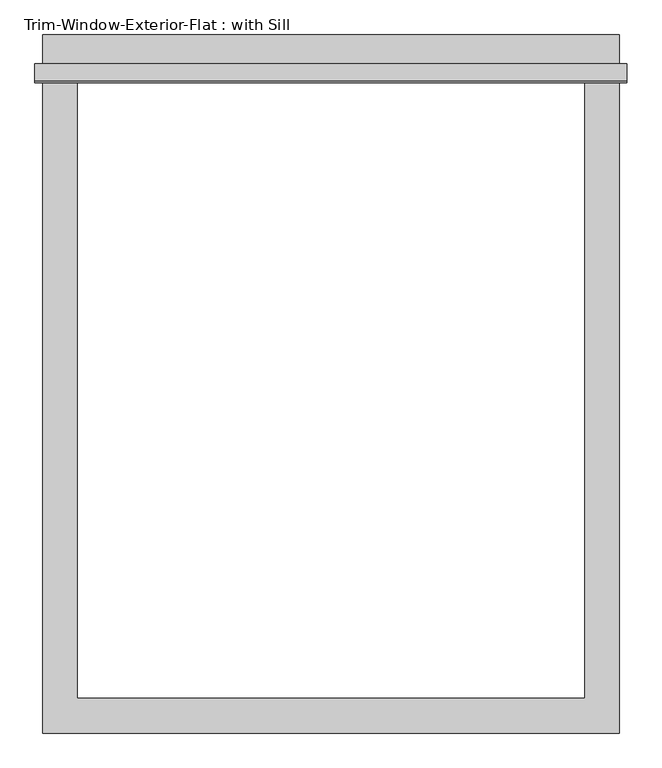
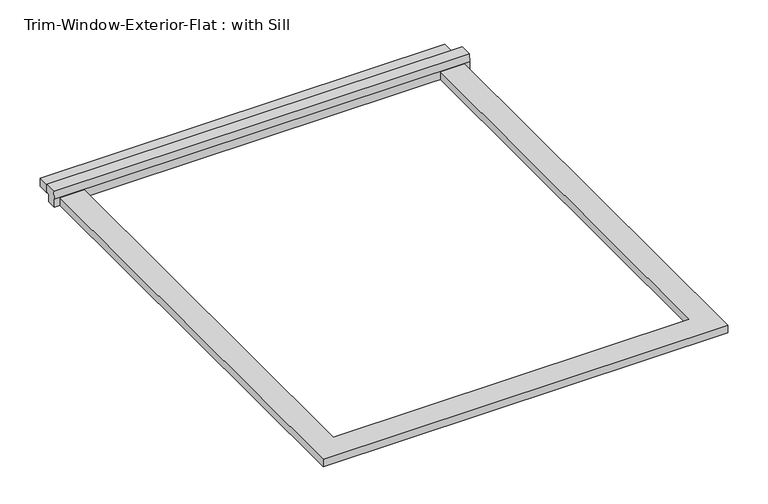
"""IFC4 building model written with IfcOpenShell, lengths in millimetres: proxy geometry, Trim-Window-Exterior-Flat : with Sill."""

from ifc_helpers import new_model, si_unit, frame, origin, origin_with_axes, place, context, project, spatial, polyline, outline, extrude, source, transform, mapped, element, save


def trim_window_exterior_flat_with_sill_92d7e9d7(model_context):
    return source(origin(), model_context, "Body", "SweptSolid", [
        extrude(outline(polyline([(476.25, 1038.1823709), (-476.25, 1038.1823709), (-476.25, 1095.3323709), (476.25, 1095.3323709), (476.25, 1038.1823709)])), origin_with_axes(), (0.0, 0.0, 1.0), 19.05),
        extrude(outline(polyline([(1047.75, 38.1), (1047.75, 19.05), (1038.1823709, 19.05), (1038.1823709, 0.0), (1016.0, 0.0), (1016.0, 19.05), (1018.4580645, 38.1), (1047.75, 38.1)])), frame((-488.95, 0.0, 0.0), z_axis=(1.0, 0.0, 0.0), x_axis=(0.0, 1.0, 0.0)), (0.0, 0.0, 1.0), 977.9),
        extrude(outline(polyline([(-476.25, -57.15), (-476.25, 1016.0), (-419.1, 1016.0), (-419.1, 0.0), (419.1, 0.0), (419.1, 1016.0), (476.25, 1016.0), (476.25, -57.15), (-476.25, -57.15)])), origin_with_axes(), (0.0, 0.0, 1.0), 19.05),
    ])


if __name__ == "__main__":
    model = new_model("IFC4")
    model_context = context("Model", 3, world=origin())
    ifc_project = project(units=[si_unit("LENGTHUNIT", "METRE", prefix="MILLI")], contexts=[model_context])
    site = spatial("IfcSite", under=ifc_project)
    building = spatial("IfcBuilding", under=site)
    placement = place(None, origin())
    trim_window_exterior_flat_with_sill_shape = trim_window_exterior_flat_with_sill_92d7e9d7(model_context)
    element("IfcBuildingElementProxy", 1, Name="Trim-Window-Exterior-Flat : with Sill", ObjectType="Trim-Window-Exterior-Flat : with Sill", at=placement, inside=building, context=model_context, shape_type="MappedRepresentation", body=[
        mapped(trim_window_exterior_flat_with_sill_shape, transform((0.0, 0.0, 0.0), x_axis=(1.0, 0.0, 0.0), y_axis=(0.0, 1.0, 0.0), z_axis=(0.0, 0.0, 1.0))),
    ])
    save(model, "model.ifc")

# Revit data of these elements
# Type "Trim-Window-Exterior-Flat : with Sill"
#   Trim Width = 0' - 2 1/4"
#   Trim Thickness_Picture Frame = 0' - 1 1/4"
#   Trim Thickness_with Sill = 0' - 0 3/4"
#   Sill Thickness = 0' - 1 1/4"
#   Opening Width [instance default] = 2' - 0"
#   Opening Height [instance default] = 3' - 0"
#   Default Elevation = 4' - 0"
#   Sill = yes
#   Picture Frame = no
#   Trim Material [instance default] = none
# Element 1 (IfcBuildingElementProxy, "Trim-Window-Exterior-Flat : with Sill")
#   Opening Width = 2' - 9"
#   Opening Height = 3' - 4"
#   Trim Material = Clad - White
#   Materials on its faces: "Clad - White"
# Materials
#   "Clad - White": class "Wood", colour RGB 242 242 238, transparency 0, Cost = 0
